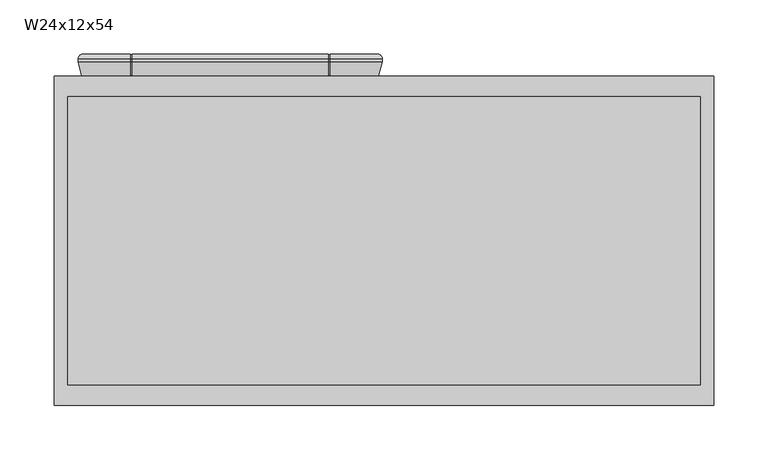
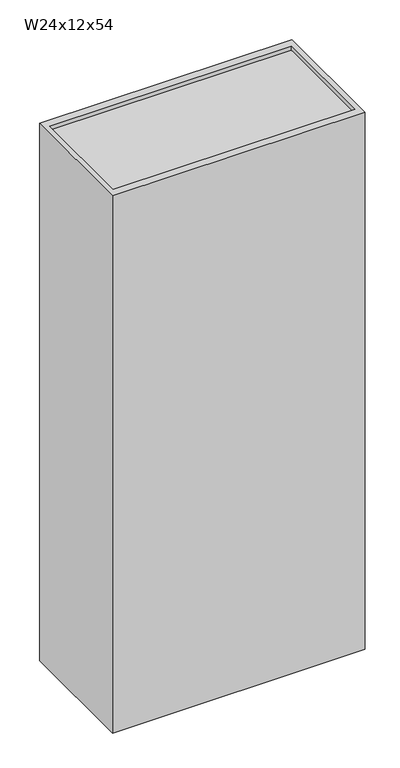
"""IFC4 building model written with IfcOpenShell, lengths in millimetres: furniture geometry, Cabinet-Wall-Merillat-Double_Door-Marlin : W24x12x54."""

from ifc_helpers import new_model, si_unit, frame, origin, place, context, project, spatial, polyline, circle_curve, ellipse_curve, outline, extrude, faceted_brep, source, transform, mapped, element, save
from ifc_brep_helpers import plane_surface, cylinder_surface, advanced_brep


def w24x12x54_50b2b19f(model_context):
    return source(origin(), model_context, "Body", "SolidModel", [
        advanced_brep(
        [(-24.0971608, 401.6121, 2108.2), (-21.0006683, 406.0825, 2105.1035075), (-21.0006683, 406.0825, 790.4964925), (-24.0971608, 401.6121, 787.4), (-24.0971608, 398.8435, 787.4), (-24.0971608, 398.8435, 2108.2), (-20.5919608, 385.7625, 790.9052), (-20.5919608, 385.7625, 2104.6948), (24.104002, 385.7625, 2059.9988372), (24.104002, 385.7625, 835.6011628), (24.4741337, 386.55625, 835.9712945), (26.5552927, 391.01931, 838.0524535), (26.5552927, 391.01931, 2057.5475465), (24.4741337, 386.55625, 2059.6287055), (25.1555233, 393.2594093, 836.652684), (25.1555233, 393.2594093, 2058.947316), (10.8278392, 393.5095, 822.325), (10.8278392, 393.5095, 2073.275), (10.8278392, 398.3355, 822.325), (10.8278392, 398.3355, 2073.275), (25.1555233, 398.5855907, 836.652684), (25.1555233, 398.5855907, 2058.947316), (26.5552927, 400.82569, 838.0524535), (26.5552927, 400.82569, 2057.5475465), (24.4741337, 405.28875, 835.9712945), (24.1068694, 406.0763508, 835.6040302), (24.104002, 406.0825, 2059.9988372), (24.4741337, 405.28875, 2059.6287055), (24.1068694, 406.0825, 790.4964925), (24.1068694, 401.6121, 787.4), (253.7938467, 406.0825, 790.4964925), (256.8903392, 401.6121, 787.4), (208.7261206, 401.6121, 787.4), (208.7261206, 406.0825, 790.4964925), (25.6943694, 401.6121, 787.4), (25.6943694, 406.0825, 790.4964925), (207.1386206, 406.0825, 790.4964925), (207.1386206, 401.6121, 787.4), (24.1068694, 398.8435, 787.4), (256.8903392, 398.8435, 787.4), (208.7261206, 398.8435, 787.4), (25.6943694, 398.8435, 787.4), (207.1386206, 398.8435, 787.4), (24.1068694, 385.7625, 790.9052), (253.3851392, 385.7625, 790.9052), (208.7261206, 385.7625, 790.9052), (25.6943694, 385.7625, 790.9052), (207.1386206, 385.7625, 790.9052), (206.2378857, 391.01931, 838.0524535), (25.6943694, 386.55625, 835.9712945), (25.6943694, 385.7625, 835.6011628), (207.1386206, 385.7625, 835.6011628), (207.1386206, 386.55625, 835.9712945), (208.3190448, 386.55625, 835.9712945), (207.6376552, 393.2594093, 836.652684), (221.9653392, 393.5095, 822.325), (221.9653392, 398.3355, 822.325), (207.6376552, 398.5855907, 836.652684), (206.2378857, 400.82569, 838.0524535), (208.3190448, 405.28875, 835.9712945), (207.1386206, 405.28875, 835.9712945), (207.1386206, 406.0825, 835.6011628), (25.6943694, 406.0825, 835.6011628), (25.6943694, 405.28875, 835.9712945), (253.7938467, 406.0825, 2105.1035075), (256.8903392, 401.6121, 2108.2), (256.8903392, 398.8435, 2108.2), (253.3851392, 385.7625, 2104.6948), (208.6891765, 385.7625, 835.6011628), (208.6891765, 385.7625, 2059.9988372), (208.3190448, 386.55625, 2059.6287055), (206.2378857, 391.01931, 2057.5475465), (207.6376552, 393.2594093, 2058.947316), (221.9653392, 393.5095, 2073.275), (221.9653392, 398.3355, 2073.275), (207.6376552, 398.5855907, 2058.947316), (206.2378857, 400.82569, 2057.5475465), (208.3190448, 405.28875, 2059.6287055), (208.6891765, 406.0825, 2059.9988372), (208.6891765, 406.0825, 835.6011628), (208.7261206, 406.0825, 2105.1035075), (208.7261206, 401.6121, 2108.2), (24.1068694, 401.6121, 2108.2), (24.1068694, 406.0825, 2105.1035075), (207.1386206, 401.6121, 2108.2), (207.1386206, 406.0825, 2105.1035075), (25.6943694, 406.0825, 2105.1035075), (25.6943694, 401.6121, 2108.2), (208.7261206, 398.8435, 2108.2), (24.1068694, 398.8435, 2108.2), (207.1386206, 398.8435, 2108.2), (25.6943694, 398.8435, 2108.2), (208.7261206, 385.7625, 2104.6948), (24.1068694, 385.7625, 2104.6948), (207.1386206, 385.7625, 2104.6948), (25.6943694, 385.7625, 2104.6948), (207.1386206, 385.7625, 2059.9988372), (25.6943694, 385.7625, 2059.9988372), (207.1386206, 386.55625, 2059.6287055), (25.6943694, 386.55625, 2059.6287055), (25.6943694, 405.28875, 2059.6287055), (25.6943694, 406.0825, 2059.9988372), (207.1386206, 406.0825, 2059.9988372), (207.1386206, 405.28875, 2059.6287055), (207.1386206, 386.55625, 2104.0857412), (207.1386206, 398.9480037, 2107.40625), (207.1386206, 401.6121, 2107.40625), (207.1386206, 405.28875, 2104.9526052), (208.7261206, 405.28875, 2059.6287055), (208.7261206, 405.28875, 2104.9526052), (208.7261206, 401.6121, 2107.40625), (208.7261206, 398.9480037, 2107.40625), (208.7261206, 386.55625, 2104.0857412), (208.7261206, 386.55625, 2059.6287055), (24.1068694, 386.55625, 2059.6287055), (24.1068694, 386.55625, 2104.0857412), (24.1068694, 398.9480037, 2107.40625), (24.1068694, 401.6121, 2107.40625), (24.1068694, 405.28875, 2104.9526052), (24.1068694, 405.28875, 2059.6287055), (25.6943694, 405.28875, 2104.9526052), (25.6943694, 401.6121, 2107.40625), (25.6943694, 398.9480037, 2107.40625), (25.6943694, 386.55625, 2104.0857412), (24.1068694, 405.28875, 835.9712945), (24.1068694, 405.28875, 790.6473948), (24.1068694, 401.6121, 788.19375), (24.1068694, 398.9480037, 788.19375), (24.1068694, 386.55625, 791.5142588), (24.1068694, 386.55625, 835.9712945), (25.6943694, 386.55625, 791.5142588), (25.6943694, 398.9480037, 788.19375), (25.6943694, 401.6121, 788.19375), (25.6943694, 405.28875, 790.6473948), (207.1386206, 405.28875, 790.6473948), (207.1386206, 401.6121, 788.19375), (207.1386206, 398.9480037, 788.19375), (207.1386206, 386.55625, 791.5142588), (208.7261206, 405.28875, 835.9712945), (208.7261206, 386.55625, 835.9712945), (208.7261206, 386.55625, 791.5142588), (208.7261206, 398.9480037, 788.19375), (208.7261206, 401.6121, 788.19375), (208.7261206, 405.28875, 790.6473948)],
        [
            (0, 1, ellipse_curve(frame((-19.3219608, 401.6121, 2103.4248), z_axis=(-0.7071067811865475, 0.0, -0.7071067811865475), x_axis=(-0.7071067811865474, 0.0, 0.7071067811865476)), 6.7531526, 4.7752)),
            (1, 2),
            (2, 3, ellipse_curve(frame((-19.3219608, 401.6121, 792.1752), z_axis=(-0.7071067811865475, 0.0, 0.7071067811865475), x_axis=(0.7071067811865474, 0.0, 0.7071067811865476)), 6.7531526, 4.7752)),
            (3, 0),
            (3, 4),
            (4, 5),
            (5, 0),
            (4, 6),
            (6, 7),
            (7, 5),
            (8, 9),
            (9, 10),
            (10, 11),
            (11, 12),
            (12, 13),
            (13, 8),
            (11, 14, ellipse_curve(frame((25.1280392, 391.6848492, 836.6252), z_axis=(-0.7071067811865475, 0.0, 0.7071067811865475), x_axis=(0.7071067811865474, 0.0, 0.7071067811865476)), 2.2271035, 1.5748)),
            (14, 15),
            (15, 12, ellipse_curve(frame((25.1280392, 391.6848492, 2058.9748), z_axis=(-0.7071067811865475, 0.0, -0.7071067811865475), x_axis=(-0.7071067811865474, 0.0, 0.7071067811865476)), 2.2271035, 1.5748)),
            (14, 16),
            (16, 17),
            (17, 15),
            (16, 18),
            (18, 19),
            (19, 17),
            (18, 20),
            (20, 21),
            (21, 19),
            (20, 22, ellipse_curve(frame((25.1280392, 400.1601508, 836.6252), z_axis=(-0.7071067811865475, 0.0, 0.7071067811865475), x_axis=(0.7071067811865474, 0.0, 0.7071067811865476)), 2.2271035, 1.5748)),
            (22, 23),
            (23, 21, ellipse_curve(frame((25.1280392, 400.1601508, 2058.9748), z_axis=(-0.7071067811865475, 0.0, -0.7071067811865475), x_axis=(-0.7071067811865474, 0.0, 0.7071067811865476)), 2.2271035, 1.5748)),
            (22, 24),
            (24, 25),
            (25, 26),
            (26, 27),
            (27, 23),
            (2, 28),
            (28, 29, circle_curve(frame((24.1068694, 401.6121, 792.1752), z_axis=(-1.0, 0.0, 0.0), x_axis=(0.0, -1.0, 0.0)), 4.7752)),
            (29, 3),
            (30, 31, ellipse_curve(frame((252.1151392, 401.6121, 792.1752), z_axis=(-0.7071067811865475, 0.0, -0.7071067811865475), x_axis=(-0.7071067811865476, 0.0, 0.7071067811865474)), 6.7531526, 4.7752)),
            (31, 32),
            (32, 33, circle_curve(frame((208.7261206, 401.6121, 792.1752), z_axis=(1.0, 0.0, 0.0), x_axis=(0.0, -1.0, 0.0)), 4.7752)),
            (33, 30),
            (34, 35, circle_curve(frame((25.6943694, 401.6121, 792.1752), z_axis=(1.0, 0.0, 0.0), x_axis=(0.0, -1.0, 0.0)), 4.7752)),
            (35, 36),
            (36, 37, circle_curve(frame((207.1386206, 401.6121, 792.1752), z_axis=(-1.0, 0.0, 0.0), x_axis=(0.0, -1.0, 0.0)), 4.7752)),
            (37, 34),
            (29, 38),
            (38, 4),
            (31, 39),
            (39, 40),
            (40, 32),
            (41, 34),
            (37, 42),
            (42, 41),
            (38, 43),
            (43, 6),
            (39, 44),
            (44, 45),
            (45, 40),
            (46, 41),
            (42, 47),
            (47, 46),
            (48, 11),
            (10, 49),
            (49, 50),
            (50, 51),
            (51, 52),
            (52, 53),
            (53, 48),
            (48, 54, ellipse_curve(frame((207.6651392, 391.6848492, 836.6252), z_axis=(-0.7071067811865475, 0.0, -0.7071067811865475), x_axis=(-0.7071067811865476, 0.0, 0.7071067811865474)), 2.2271035, 1.5748)),
            (54, 14),
            (54, 55),
            (55, 16),
            (55, 56),
            (56, 18),
            (56, 57),
            (57, 20),
            (57, 58, ellipse_curve(frame((207.6651392, 400.1601508, 836.6252), z_axis=(-0.7071067811865475, 0.0, -0.7071067811865475), x_axis=(-0.7071067811865476, 0.0, 0.7071067811865474)), 2.2271035, 1.5748)),
            (58, 22),
            (58, 59),
            (59, 60),
            (60, 61),
            (61, 62),
            (62, 63),
            (63, 24),
            (30, 64),
            (64, 65, ellipse_curve(frame((252.1151392, 401.6121, 2103.4248), z_axis=(0.7071067811865475, 0.0, -0.7071067811865475), x_axis=(-0.7071067811865474, 0.0, -0.7071067811865476)), 6.7531526, 4.7752)),
            (65, 31),
            (65, 66),
            (66, 39),
            (66, 67),
            (67, 44),
            (68, 69),
            (69, 70),
            (70, 71),
            (71, 48),
            (53, 68),
            (71, 72, ellipse_curve(frame((207.6651392, 391.6848492, 2058.9748), z_axis=(0.7071067811865475, 0.0, -0.7071067811865475), x_axis=(-0.7071067811865474, 0.0, -0.7071067811865476)), 2.2271035, 1.5748)),
            (72, 54),
            (72, 73),
            (73, 55),
            (73, 74),
            (74, 56),
            (74, 75),
            (75, 57),
            (75, 76, ellipse_curve(frame((207.6651392, 400.1601508, 2058.9748), z_axis=(0.7071067811865475, 0.0, -0.7071067811865475), x_axis=(-0.7071067811865474, 0.0, -0.7071067811865476)), 2.2271035, 1.5748)),
            (76, 58),
            (76, 77),
            (77, 78),
            (78, 79),
            (79, 59),
            (64, 80),
            (80, 81, circle_curve(frame((208.7261206, 401.6121, 2103.4248), z_axis=(1.0, 0.0, 0.0), x_axis=(0.0, -1.0, 0.0)), 4.7752)),
            (81, 65),
            (0, 82),
            (82, 83, circle_curve(frame((24.1068694, 401.6121, 2103.4248), z_axis=(-1.0, 0.0, 0.0), x_axis=(0.0, -1.0, 0.0)), 4.7752)),
            (83, 1),
            (84, 85, circle_curve(frame((207.1386206, 401.6121, 2103.4248), z_axis=(-1.0, 0.0, 0.0), x_axis=(0.0, -1.0, 0.0)), 4.7752)),
            (85, 86),
            (86, 87, circle_curve(frame((25.6943694, 401.6121, 2103.4248), z_axis=(1.0, 0.0, 0.0), x_axis=(0.0, -1.0, 0.0)), 4.7752)),
            (87, 84),
            (81, 88),
            (88, 66),
            (5, 89),
            (89, 82),
            (90, 84),
            (87, 91),
            (91, 90),
            (88, 92),
            (92, 67),
            (7, 93),
            (93, 89),
            (94, 90),
            (91, 95),
            (95, 94),
            (43, 9),
            (8, 93),
            (92, 69),
            (68, 45),
            (96, 94),
            (95, 97),
            (97, 96),
            (50, 46),
            (47, 51),
            (12, 71),
            (70, 98),
            (98, 96),
            (97, 99),
            (99, 13),
            (15, 72),
            (17, 73),
            (19, 74),
            (21, 75),
            (23, 76),
            (27, 100),
            (100, 101),
            (101, 102),
            (102, 103),
            (103, 77),
            (83, 26),
            (25, 28),
            (33, 79),
            (78, 80),
            (85, 102),
            (101, 86),
            (35, 62),
            (61, 36),
            (98, 104),
            (104, 105),
            (105, 106),
            (106, 107, circle_curve(frame((207.1386206, 401.6121, 2103.4248), z_axis=(-1.0, 0.0, 0.0), x_axis=(0.0, 0.0, 1.0)), 3.98145)),
            (107, 103),
            (78, 108),
            (108, 109),
            (109, 110, circle_curve(frame((208.7261206, 401.6121, 2103.4248), z_axis=(1.0, 0.0, 0.0), x_axis=(0.0, 0.0, 1.0)), 3.98145)),
            (110, 111),
            (111, 112),
            (112, 113),
            (113, 69),
            (77, 108),
            (107, 109),
            (106, 110),
            (105, 111),
            (104, 112),
            (70, 113),
            (8, 114),
            (114, 115),
            (115, 116),
            (116, 117),
            (117, 118, circle_curve(frame((24.1068694, 401.6121, 2103.4248), z_axis=(-1.0, 0.0, 0.0), x_axis=(0.0, 0.0, 1.0)), 3.98145)),
            (118, 119),
            (119, 26),
            (100, 120),
            (120, 121, circle_curve(frame((25.6943694, 401.6121, 2103.4248), z_axis=(1.0, 0.0, 0.0), x_axis=(0.0, 0.0, 1.0)), 3.98145)),
            (121, 122),
            (122, 123),
            (123, 99),
            (119, 27),
            (118, 120),
            (117, 121),
            (116, 122),
            (115, 123),
            (114, 13),
            (25, 124),
            (124, 125),
            (125, 126, circle_curve(frame((24.1068694, 401.6121, 792.1752), z_axis=(-1.0, 0.0, 0.0), x_axis=(0.0, 0.0, 1.0)), 3.98145)),
            (126, 127),
            (127, 128),
            (128, 129),
            (129, 9),
            (49, 130),
            (130, 131),
            (131, 132),
            (132, 133, circle_curve(frame((25.6943694, 401.6121, 792.1752), z_axis=(1.0, 0.0, 0.0), x_axis=(0.0, 0.0, 1.0)), 3.98145)),
            (133, 63),
            (129, 10),
            (128, 130),
            (127, 131),
            (126, 132),
            (125, 133),
            (124, 24),
            (60, 134),
            (134, 135, circle_curve(frame((207.1386206, 401.6121, 792.1752), z_axis=(-1.0, 0.0, 0.0), x_axis=(0.0, 0.0, 1.0)), 3.98145)),
            (135, 136),
            (136, 137),
            (137, 52),
            (138, 79),
            (68, 139),
            (139, 140),
            (140, 141),
            (141, 142),
            (142, 143, circle_curve(frame((208.7261206, 401.6121, 792.1752), z_axis=(1.0, 0.0, 0.0), x_axis=(0.0, 0.0, 1.0)), 3.98145)),
            (143, 138),
            (138, 59),
            (53, 139),
            (137, 140),
            (136, 141),
            (135, 142),
            (134, 143),
        ],
        [
            cylinder_surface(frame((-19.3219608, 401.6121, 2108.2), z_axis=(0.0, 0.0, 1.0), x_axis=(0.0, -1.0, 0.0)), 4.7752),
            plane_surface(frame((-24.0971608, 401.6121, 2108.2), z_axis=(-1.0, 0.0, 0.0), x_axis=(0.0, 0.0, -1.0))),
            plane_surface(frame((-24.0971608, 398.8435, 2108.2), z_axis=(-0.9659229350723619, -0.25882983502910506, 0.0), x_axis=(0.0, 0.0, -1.0))),
            plane_surface(frame((24.104002, 385.7625, 2059.9988372), z_axis=(0.9063077870366099, -0.4226182617407856, 0.0), x_axis=(0.0, 0.0, -1.0))),
            cylinder_surface(frame((25.1280392, 391.6848492, 2108.2), z_axis=(0.0, 0.0, 1.0000000000000002), x_axis=(0.01745240643729364, 0.9998476951563912, 0.0)), 1.5748),
            plane_surface(frame((25.1555233, 393.2594093, 2058.947316), z_axis=(0.017452406437322144, 0.9998476951563906, 0.0), x_axis=(0.0, 0.0, -1.0))),
            plane_surface(frame((10.8278392, 393.5095, 2073.275), z_axis=(1.0, 0.0, 0.0), x_axis=(0.0, 0.0, -1.0))),
            plane_surface(frame((10.8278392, 398.3355, 2073.275), z_axis=(0.01745240643727848, -0.9998476951563914, 0.0), x_axis=(0.0, 0.0, -1.0))),
            cylinder_surface(frame((25.1280392, 400.1601508, 2108.2), z_axis=(0.0, 0.0, 1.0000000000000002), x_axis=(0.9063077870367326, 0.42261826174052236, 0.0)), 1.5748),
            plane_surface(frame((26.5552927, 400.82569, 2057.5475465), z_axis=(0.9063077870366333, 0.4226182617407352, 0.0), x_axis=(0.0, 0.0, -1.0))),
            cylinder_surface(frame((-24.0971608, 401.6121, 792.1752), z_axis=(-1.0, 0.0, 0.0), x_axis=(0.0, -1.0, 0.0)), 4.7752),
            plane_surface(frame((-24.0971608, 401.6121, 787.4), z_axis=(0.0, 0.0, -1.0), x_axis=(1.0, 0.0, 0.0))),
            plane_surface(frame((-24.0971608, 398.8435, 787.4), z_axis=(0.0, -0.2588298350291095, -0.9659229350723607), x_axis=(1.0, 0.0, 0.0))),
            plane_surface(frame((24.104002, 385.7625, 835.6011628), z_axis=(0.0, -0.42261826174078143, 0.9063077870366119), x_axis=(1.0, 0.0, 0.0))),
            cylinder_surface(frame((-24.0971608, 391.6848492, 836.6252), z_axis=(-1.0000000000000002, 0.0, 0.0), x_axis=(0.0, 0.9998476951563913, 0.017452406437289025)), 1.5748),
            plane_surface(frame((25.1555233, 393.2594093, 836.652684), z_axis=(0.0, 0.9998476951563907, 0.01745240643731753), x_axis=(1.0, 0.0, 0.0))),
            plane_surface(frame((10.8278392, 393.5095, 822.325), z_axis=(0.0, 0.0, 1.0), x_axis=(1.0, 0.0, 0.0))),
            plane_surface(frame((10.8278392, 398.3355, 822.325), z_axis=(0.0, -0.9998476951563913, 0.017452406437283095), x_axis=(1.0, 0.0, 0.0))),
            cylinder_surface(frame((-24.0971608, 400.1601508, 836.6252), z_axis=(-1.0000000000000002, 0.0, 0.0), x_axis=(0.0, 0.4226182617405265, 0.9063077870367306)), 1.5748),
            plane_surface(frame((26.5552927, 400.82569, 838.0524535), z_axis=(0.0, 0.4226182617407394, 0.9063077870366314), x_axis=(1.0, 0.0, 0.0))),
            cylinder_surface(frame((252.1151392, 401.6121, 787.4), z_axis=(0.0, 0.0, -1.0), x_axis=(0.0, -1.0, 0.0)), 4.7752),
            plane_surface(frame((256.8903392, 401.6121, 787.4), z_axis=(1.0, 0.0, 0.0), x_axis=(0.0, 0.0, 1.0))),
            plane_surface(frame((256.8903392, 398.8435, 787.4), z_axis=(0.9659229350723619, -0.25882983502910506, 0.0), x_axis=(0.0, 0.0, 1.0))),
            plane_surface(frame((208.6891765, 385.7625, 835.6011628), z_axis=(-0.9063077870366099, -0.4226182617407856, 0.0), x_axis=(0.0, 0.0, 1.0))),
            cylinder_surface(frame((207.6651392, 391.6848492, 787.4), z_axis=(0.0, 0.0, -1.0000000000000002), x_axis=(-0.01745240643729364, 0.9998476951563912, 0.0)), 1.5748),
            plane_surface(frame((207.6376552, 393.2594093, 836.652684), z_axis=(-0.017452406437322144, 0.9998476951563906, 0.0), x_axis=(0.0, 0.0, 1.0))),
            plane_surface(frame((221.9653392, 393.5095, 822.325), z_axis=(-1.0, 0.0, 0.0), x_axis=(0.0, 0.0, 1.0))),
            plane_surface(frame((221.9653392, 398.3355, 822.325), z_axis=(-0.01745240643727848, -0.9998476951563914, 0.0), x_axis=(0.0, 0.0, 1.0))),
            cylinder_surface(frame((207.6651392, 400.1601508, 787.4), z_axis=(0.0, 0.0, -1.0000000000000002), x_axis=(-0.9063077870367326, 0.42261826174052236, 0.0)), 1.5748),
            plane_surface(frame((206.2378857, 400.82569, 838.0524535), z_axis=(-0.9063077870366333, 0.4226182617407352, 0.0), x_axis=(0.0, 0.0, 1.0))),
            cylinder_surface(frame((256.8903392, 401.6121, 2103.4248), z_axis=(1.0, 0.0, 0.0), x_axis=(0.0, -1.0, 0.0)), 4.7752),
            plane_surface(frame((256.8903392, 401.6121, 2108.2), z_axis=(0.0, 0.0, 1.0), x_axis=(-1.0, 0.0, 0.0))),
            plane_surface(frame((256.8903392, 398.8435, 2108.2), z_axis=(0.0, -0.2588298350291006, 0.9659229350723632), x_axis=(-1.0, 0.0, 0.0))),
            plane_surface(frame((253.3851392, 385.7625, 2104.6948), z_axis=(0.0, -1.0, 0.0), x_axis=(-1.0, 0.0, 0.0))),
            plane_surface(frame((208.6891765, 385.7625, 2059.9988372), z_axis=(0.0, -0.42261826174078976, -0.9063077870366079), x_axis=(-1.0, 0.0, 0.0))),
            cylinder_surface(frame((256.8903392, 391.6848492, 2058.9748), z_axis=(1.0000000000000002, 0.0, 0.0), x_axis=(0.0, 0.999847695156391, -0.017452406437298253)), 1.5748),
            plane_surface(frame((207.6376552, 393.2594093, 2058.947316), z_axis=(0.0, 0.9998476951563905, -0.01745240643732676), x_axis=(-1.0, 0.0, 0.0))),
            plane_surface(frame((221.9653392, 393.5095, 2073.275), z_axis=(0.0, 0.0, -1.0), x_axis=(-1.0, 0.0, 0.0))),
            plane_surface(frame((221.9653392, 398.3355, 2073.275), z_axis=(0.0, -0.9998476951563915, -0.017452406437273867), x_axis=(-1.0, 0.0, 0.0))),
            cylinder_surface(frame((256.8903392, 400.1601508, 2058.9748), z_axis=(1.0000000000000002, 0.0, 0.0), x_axis=(0.0, 0.4226182617405182, -0.9063077870367346)), 1.5748),
            plane_surface(frame((206.2378857, 400.82569, 2057.5475465), z_axis=(0.0, 0.422618261740731, -0.9063077870366353), x_axis=(-1.0, 0.0, 0.0))),
            plane_surface(frame((208.6891765, 406.0825, 2059.9988372), z_axis=(0.0, 1.0, 0.0), x_axis=(-1.0, 0.0, 0.0))),
            plane_surface(frame((207.1386206, 406.0825, 2059.9988372), z_axis=(1.0000000000000002, 0.0, 0.0), x_axis=(0.0, -0.9063077870366177, -0.4226182617407689))),
            plane_surface(frame((208.7261206, 406.0825, 2059.9988372), z_axis=(-1.0000000000000002, 0.0, 0.0), x_axis=(0.0, 0.9063077870366177, 0.4226182617407689))),
            plane_surface(frame((207.1386206, 406.0825, 2059.9988372), z_axis=(0.0, -0.4226182617407689, 0.9063077870366177), x_axis=(1.0, 0.0, 0.0))),
            plane_surface(frame((207.1386206, 405.28875, 2059.6287055), z_axis=(0.0, 1.0, 0.0), x_axis=(1.0, 0.0, 0.0))),
            cylinder_surface(frame((208.7261206, 401.6121, 2103.4248), z_axis=(1.0, 0.0, 0.0), x_axis=(0.0, 0.0, 1.0)), 3.98145),
            plane_surface(frame((207.1386206, 401.6121, 2107.40625), z_axis=(0.0, 0.0, 1.0), x_axis=(1.0, 0.0, 0.0))),
            plane_surface(frame((207.1386206, 398.9480037, 2107.40625), z_axis=(0.0, -0.2588298350291571, 0.965922935072348), x_axis=(1.0, 0.0, 0.0))),
            plane_surface(frame((207.1386206, 386.55625, 2104.0857412), z_axis=(0.0, -1.0, 0.0), x_axis=(1.0, 0.0, 0.0))),
            plane_surface(frame((207.1386206, 386.55625, 2059.6287055), z_axis=(0.0, 0.4226182617408151, 0.906307787036596), x_axis=(1.0, 0.0, 0.0))),
            plane_surface(frame((24.1068694, 406.0825, 2059.9988372), z_axis=(1.0, 0.0, 0.0), x_axis=(0.0, -0.9063077870366254, -0.42261826174075223))),
            plane_surface(frame((25.6943694, 406.0825, 2059.9988372), z_axis=(-1.0, 0.0, 0.0), x_axis=(0.0, 0.9063077870366254, 0.42261826174075223))),
            plane_surface(frame((24.1068694, 406.0825, 2059.9988372), z_axis=(0.0, -0.42261826174075223, 0.9063077870366254), x_axis=(1.0, 0.0, 0.0))),
            plane_surface(frame((24.1068694, 405.28875, 2059.6287055), z_axis=(0.0, 1.0, 0.0), x_axis=(1.0, 0.0, 0.0))),
            cylinder_surface(frame((25.6943694, 401.6121, 2103.4248), z_axis=(1.0, 0.0, 0.0), x_axis=(0.0, 0.0, 1.0)), 3.98145),
            plane_surface(frame((24.1068694, 401.6121, 2107.40625), z_axis=(0.0, 0.0, 1.0), x_axis=(1.0, 0.0, 0.0))),
            plane_surface(frame((24.1068694, 398.9480037, 2107.40625), z_axis=(0.0, -0.258829835029159, 0.9659229350723475), x_axis=(1.0, 0.0, 0.0))),
            plane_surface(frame((24.1068694, 386.55625, 2104.0857412), z_axis=(0.0, -1.0, 0.0), x_axis=(1.0, 0.0, 0.0))),
            plane_surface(frame((24.1068694, 386.55625, 2059.6287055), z_axis=(0.0, 0.4226182617408322, 0.9063077870365881), x_axis=(1.0, 0.0, 0.0))),
            plane_surface(frame((24.1068694, 401.6121, 796.9504), z_axis=(1.0, 0.0, 0.0), x_axis=(0.0, 1.0, 0.0))),
            plane_surface(frame((25.6943694, 401.6121, 796.9504), z_axis=(-1.0, 0.0, 0.0), x_axis=(0.0, -1.0, 0.0))),
            plane_surface(frame((24.1068694, 385.7625, 835.6011628), z_axis=(0.0, 0.4226182617407559, -0.9063077870366237), x_axis=(1.0, 0.0, 0.0))),
            plane_surface(frame((24.1068694, 386.55625, 835.9712945), z_axis=(0.0, -1.0, 0.0), x_axis=(1.0, 0.0, 0.0))),
            plane_surface(frame((24.1068694, 386.55625, 791.5142588), z_axis=(0.0, -0.25882983502944146, -0.9659229350722718), x_axis=(1.0, 0.0, 0.0))),
            plane_surface(frame((24.1068694, 398.9480037, 788.19375), z_axis=(0.0, 0.0, -1.0), x_axis=(1.0, 0.0, 0.0))),
            cylinder_surface(frame((25.6943694, 401.6121, 792.1752), z_axis=(1.0, 0.0, 0.0), x_axis=(0.0, 0.0, 1.0)), 3.98145),
            plane_surface(frame((24.1068694, 405.28875, 790.6473948), z_axis=(0.0, 1.0, 0.0), x_axis=(1.0, 0.0, 0.0))),
            plane_surface(frame((24.1068694, 405.28875, 835.9712945), z_axis=(0.0, -0.42261826174073325, -0.9063077870366342), x_axis=(1.0, 0.0, 0.0))),
            plane_surface(frame((207.1386206, 405.28875, 835.9712945), z_axis=(1.0, 0.0, 0.0), x_axis=(0.0, 0.9063077870366539, -0.42261826174069095))),
            plane_surface(frame((208.7261206, 405.28875, 835.9712945), z_axis=(-1.0, 0.0, 0.0), x_axis=(0.0, -0.9063077870366539, 0.42261826174069095))),
            plane_surface(frame((207.1386206, 405.28875, 835.9712945), z_axis=(0.0, -0.42261826174069095, -0.9063077870366539), x_axis=(1.0, 0.0, 0.0))),
            plane_surface(frame((207.1386206, 385.7625, 835.6011628), z_axis=(0.0, 0.42261826174079387, -0.9063077870366061), x_axis=(1.0, 0.0, 0.0))),
            plane_surface(frame((207.1386206, 386.55625, 835.9712945), z_axis=(0.0, -1.0, 0.0), x_axis=(1.0, 0.0, 0.0))),
            plane_surface(frame((207.1386206, 386.55625, 791.5142588), z_axis=(0.0, -0.25882983502944, -0.9659229350722722), x_axis=(1.0, 0.0, 0.0))),
            plane_surface(frame((207.1386206, 398.9480037, 788.19375), z_axis=(0.0, 0.0, -1.0), x_axis=(1.0, 0.0, 0.0))),
            cylinder_surface(frame((208.7261206, 401.6121, 792.1752), z_axis=(1.0, 0.0, 0.0), x_axis=(0.0, 0.0, 1.0)), 3.98145),
            plane_surface(frame((207.1386206, 405.28875, 790.6473948), z_axis=(0.0, 1.0, 0.0), x_axis=(1.0, 0.0, 0.0))),
        ],
        [
            (0, [[1, 2, 3, 4]]),
            (1, [[-4, 5, 6, 7]]),
            (2, [[-6, 8, 9, 10]]),
            (3, [[11, 12, 13, 14, 15, 16]]),
            (4, [[-14, 17, 18, 19]]),
            (5, [[-18, 20, 21, 22]]),
            (6, [[-21, 23, 24, 25]]),
            (7, [[-24, 26, 27, 28]]),
            (8, [[-27, 29, 30, 31]]),
            (9, [[-30, 32, 33, 34, 35, 36]]),
            (10, [[-3, 37, 38, 39]]),
            (10, [[40, 41, 42, 43]]),
            (10, [[44, 45, 46, 47]]),
            (11, [[-5, -39, 48, 49]]),
            (11, [[50, 51, 52, -41]]),
            (11, [[53, -47, 54, 55]]),
            (12, [[-8, -49, 56, 57]]),
            (12, [[58, 59, 60, -51]]),
            (12, [[61, -55, 62, 63]]),
            (13, [[64, -13, 65, 66, 67, 68, 69, 70]]),
            (14, [[-17, -64, 71, 72]]),
            (15, [[-20, -72, 73, 74]]),
            (16, [[-23, -74, 75, 76]]),
            (17, [[-26, -76, 77, 78]]),
            (18, [[-29, -78, 79, 80]]),
            (19, [[-80, 81, 82, 83, 84, 85, 86, -32]]),
            (20, [[-40, 87, 88, 89]]),
            (21, [[-50, -89, 90, 91]]),
            (22, [[-58, -91, 92, 93]]),
            (23, [[94, 95, 96, 97, -70, 98]]),
            (24, [[-71, -97, 99, 100]]),
            (25, [[-73, -100, 101, 102]]),
            (26, [[-75, -102, 103, 104]]),
            (27, [[-77, -104, 105, 106]]),
            (28, [[-79, -106, 107, 108]]),
            (29, [[-108, 109, 110, 111, 112, -81]]),
            (30, [[-88, 113, 114, 115]]),
            (30, [[-1, 116, 117, 118]]),
            (30, [[119, 120, 121, 122]]),
            (31, [[-90, -115, 123, 124]]),
            (31, [[-7, 125, 126, -116]]),
            (31, [[127, -122, 128, 129]]),
            (32, [[-92, -124, 130, 131]]),
            (32, [[-10, 132, 133, -125]]),
            (32, [[134, -129, 135, 136]]),
            (33, [[-9, -57, 137, -11, 138, -132]]),
            (33, [[-93, -131, 139, -94, 140, -59]]),
            (33, [[141, -136, 142, 143]]),
            (33, [[144, -63, 145, -67]]),
            (34, [[146, -96, 147, 148, -143, 149, 150, -15]]),
            (35, [[-19, 151, -99, -146]]),
            (36, [[-22, 152, -101, -151]]),
            (37, [[-25, 153, -103, -152]]),
            (38, [[-28, 154, -105, -153]]),
            (39, [[-31, 155, -107, -154]]),
            (40, [[-155, -36, 156, 157, 158, 159, 160, -109]]),
            (41, [[-2, -118, 161, -34, 162, -37]]),
            (41, [[-87, -43, 163, -111, 164, -113]]),
            (41, [[165, -158, 166, -120]]),
            (41, [[167, -84, 168, -45]]),
            (42, [[169, 170, 171, 172, 173, -159, -165, -119, -127, -134, -141, -148]]),
            (43, [[174, 175, 176, 177, 178, 179, 180, -139, -130, -123, -114, -164]]),
            (44, [[-174, -110, 181]]),
            (45, [[-173, 182, -175, -181, -160]]),
            (46, [[-172, 183, -176, -182]]),
            (47, [[-171, 184, -177, -183]]),
            (48, [[-170, 185, -178, -184]]),
            (49, [[-169, -147, 186, -179, -185]]),
            (50, [[-180, -186, -95]]),
            (51, [[187, 188, 189, 190, 191, 192, 193, -161, -117, -126, -133, -138]]),
            (52, [[194, 195, 196, 197, 198, -149, -142, -135, -128, -121, -166, -157]]),
            (53, [[-193, 199, -35]]),
            (54, [[-192, 200, -194, -156, -199]]),
            (55, [[-191, 201, -195, -200]]),
            (56, [[-190, 202, -196, -201]]),
            (57, [[-189, 203, -197, -202]]),
            (58, [[-188, 204, -150, -198, -203]]),
            (59, [[-187, -16, -204]]),
            (60, [[205, 206, 207, 208, 209, 210, 211, -137, -56, -48, -38, -162]]),
            (61, [[212, 213, 214, 215, 216, -85, -167, -44, -53, -61, -144, -66]]),
            (62, [[-211, 217, -12]]),
            (63, [[-210, 218, -212, -65, -217]]),
            (64, [[-209, 219, -213, -218]]),
            (65, [[-208, 220, -214, -219]]),
            (66, [[-207, 221, -215, -220]]),
            (67, [[-206, 222, -86, -216, -221]]),
            (68, [[-205, -33, -222]]),
            (69, [[223, 224, 225, 226, 227, -68, -145, -62, -54, -46, -168, -83]]),
            (70, [[228, -163, -42, -52, -60, -140, 229, 230, 231, 232, 233, 234]]),
            (71, [[-228, 235, -112]]),
            (72, [[-229, -98, 236]]),
            (73, [[-227, 237, -230, -236, -69]]),
            (74, [[-226, 238, -231, -237]]),
            (75, [[-225, 239, -232, -238]]),
            (76, [[-224, 240, -233, -239]]),
            (77, [[-223, -82, -235, -234, -240]]),
        ],
    ),
        extrude(outline(polyline([(221.9653392, 398.3355), (221.9653392, 393.5095), (10.8278392, 393.5095), (10.8278392, 398.3355), (221.9653392, 398.3355)])), frame((0.0, 0.0, 822.325), z_axis=(0.0, 0.0, 1.0), x_axis=(1.0, 0.0, 0.0)), (0.0, 0.0, 1.0), 1250.95),
        extrude(outline(polyline([(-8.5711577, 366.7125), (525.0128185, 366.7125), (525.0128185, 100.0125), (-8.5711577, 100.0125), (-8.5711577, 366.7125)])), frame((0.0, 0.0, 1800.225), z_axis=(0.0, 0.0, 1.0), x_axis=(1.0, 0.0, 0.0)), (0.0, 0.0, 1.0), 19.05),
        extrude(outline(polyline([(-8.5711577, 366.7125), (525.0128185, 366.7125), (525.0128185, 100.0125), (-8.5711577, 100.0125), (-8.5711577, 366.7125)])), frame((0.0, 0.0, 1076.325), z_axis=(0.0, 0.0, 1.0), x_axis=(1.0, 0.0, 0.0)), (0.0, 0.0, 1.0), 19.05),
        extrude(outline(polyline([(-8.5711577, 366.7125), (525.0128185, 366.7125), (525.0128185, 100.0125), (-8.5711577, 100.0125), (-8.5711577, 366.7125)])), frame((0.0, 0.0, 1438.275), z_axis=(0.0, 0.0, 1.0), x_axis=(1.0, 0.0, 0.0)), (0.0, 0.0, 1.0), 19.05),
        faceted_brep([(-46.3221608, 80.9625, 2133.6), (-46.3221608, 80.9625, 762.0), (563.2778392, 80.9625, 762.0), (563.2778392, 80.9625, 2133.6), (-46.3221608, 385.7625, 2133.6), (563.2778392, 385.7625, 2133.6), (563.2778392, 385.7625, 762.0), (-46.3221608, 385.7625, 762.0), (525.0128185, 385.7625, 2095.2735163), (301.9690685, 385.7625, 2095.2735163), (301.9690685, 385.7625, 799.8672696), (525.0128185, 385.7625, 799.8672696), (-8.5711577, 385.7625, 2095.2735163), (-8.5711577, 385.7625, 799.8672696), (214.98661, 385.7625, 799.8672696), (214.98661, 385.7625, 2095.2735163), (-33.6221608, 100.0125, 762.0), (550.5778392, 100.0125, 762.0), (550.5778392, 366.7125, 762.0), (-33.6221608, 366.7125, 762.0), (550.5778392, 366.7125, 2133.6), (550.5778392, 100.0125, 2133.6), (-33.6221608, 100.0125, 2133.6), (-33.6221608, 366.7125, 2133.6), (-8.5711577, 100.0125, 2095.2735163), (214.98661, 366.7125, 2095.2735163), (301.9690685, 366.7125, 2095.2735163), (525.0128185, 100.0125, 2095.2735163), (525.0128185, 100.0125, 799.8672696), (301.9690685, 366.7125, 799.8672696), (214.98661, 366.7125, 799.8672696), (-8.5711577, 100.0125, 799.8672696), (550.5778392, 100.0125, 2122.9851371), (550.5778392, 366.7125, 2122.9851371), (-33.6221608, 366.7125, 2122.9851371), (-33.6221608, 100.0125, 2122.9851371), (-33.6221608, 100.0125, 771.8352657), (-33.6221608, 366.7125, 771.8352657), (550.5778392, 366.7125, 771.8352657), (550.5778392, 100.0125, 771.8352657)], [[[0, 1, 2, 3]], [[4, 5, 6, 7], [8, 9, 10, 11], [12, 13, 14, 15]], [[1, 0, 4, 7]], [[2, 1, 7, 6], [16, 17, 18, 19]], [[3, 2, 6, 5]], [[0, 3, 5, 4], [20, 21, 22, 23]], [[24, 12, 15, 25, 26, 9, 8, 27]], [[8, 11, 28, 27]], [[28, 11, 10, 29, 30, 14, 13, 31]], [[13, 12, 24, 31]], [[32, 33, 34, 35]], [[33, 32, 21, 20]], [[34, 33, 20, 23]], [[35, 34, 23, 22]], [[32, 35, 22, 21]], [[36, 37, 38, 39]], [[36, 39, 17, 16]], [[39, 38, 18, 17]], [[38, 37, 19, 18]], [[37, 36, 16, 19]], [[24, 27, 28, 31]], [[26, 29, 10, 9]], [[15, 14, 30, 25]], [[29, 26, 25, 30]]]),
    ])


if __name__ == "__main__":
    model = new_model("IFC4")
    model_context = context("Model", 3, world=origin())
    ifc_project = project(units=[si_unit("LENGTHUNIT", "METRE", prefix="MILLI")], contexts=[model_context])
    site = spatial("IfcSite", under=ifc_project)
    building = spatial("IfcBuilding", under=site)
    placement = place(None, origin())
    w24x12x54_shape = w24x12x54_50b2b19f(model_context)
    element("IfcFurniture", 1, ObjectType="Cabinet-Wall-Merillat-Double_Door-Marlin : W24x12x54", at=placement, inside=building, context=model_context, shape_type="MappedRepresentation", body=[
        mapped(w24x12x54_shape, transform((0.0, 0.0, 0.0), x_axis=(1.0, 0.0, 0.0), y_axis=(0.0, 1.0, 0.0), z_axis=(0.0, 0.0, 1.0))),
    ])
    save(model, "model.ifc")

# Revit data of these elements
# Type "Cabinet-Wall-Merillat-Double_Door-Marlin : W24x12x54"
#   URL = "https://www.merillat.com/"
#   Product Page URL = "https://www.merillat.com/our-products/"
#   Product Line = "Express"
#   Product Group = "Wall Cabinet"
#   Product Documentation Link = "http://merillatbusiness.com/wp-content/uploads/2014/07/Merillat_Classic_Catalog.pdf"
#   Model = "W2442B"
#   Manufacturer = "Merillat"
#   Height Note = "Actual Height of 21 inches Cabinet is 20 1/2 inches"
#   Glass Door Note = "Glass Cabinet doors are only available in specific sizes. Please refer to the catalog for this information before requesting a glass size."
#   Finish = "Wood"
#   Description = "Wall 2442 Butt Door"
#   Construction Type = "Wall Cabinet"
#   Cabinet Construction Note = "Cabinets with B suffix have BUTT doors without a center frame stile:"
#   Assembly Code = "C1030410"
#   Spacing = 0' - 1"
#   Shelving Height = 1' - 0 3/4"
#   Door Spacing = 0' - 0 1/8"
#   Cabinet Door Width = 0' - 11 1/16"
#   Cabinet Door Height = 4' - 4"
#   Depth = 1' - 0"
#   Height = 4' - 6"
#   Top Of Cabinet = 7' - 0"
#   Width = 2' - 0"
#   COBie.Type = no
#   Top and Bottom Visibility = yes
#   Partial Overlay Butt = yes
#   Partial Overlay = no
#   Number of Shelves Greater than one = 3
#   Number of Shelves = 3
#   Middle Shelf = yes
#   Full Overlay Butt = no
#   Full Overlay = no
#   Elevation Swing Line = yes
#   Door Drawer Material = Wood - Merillat - Pecan(1)
#   Cabinet Material = Wood - Merillat - Pecan(1)
#   Cabinet Door Style = element 806847
# Element 1 (IfcFurniture, "Cabinet-Wall-Merillat-Double_Door-Marlin : W24x12x54")
#   Materials on its faces: "Wood - Merillat - Pecan(1)"
# Materials
#   "Wood - Merillat - Pecan(1)": class "Wood", colour RGB 108 67 43, transparency 0, Cost = 0
